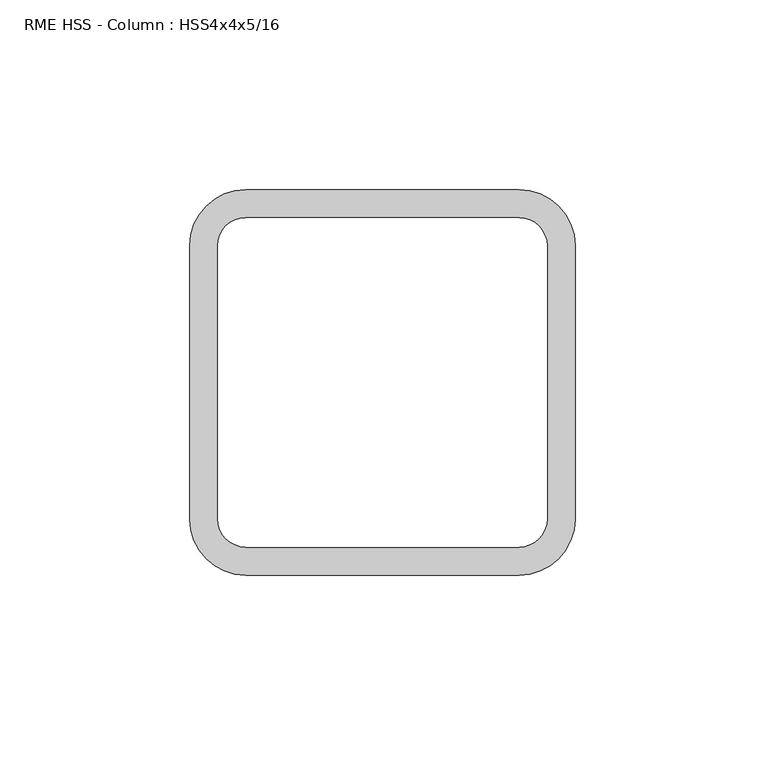
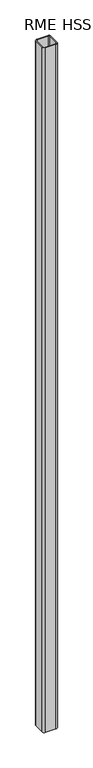
"""IFC4 building model written with IfcOpenShell, lengths in millimetres: column geometry, RME HSS - Column : HSS4x4x5/16."""

import ifcopenshell
import ifcopenshell.guid

model = None  # the IFC model being written
_history = None  # IfcOwnerHistory: only IFC2X3 demands one
_inside = {}  # id of a spatial element -> (the spatial element, [elements in it])
_under = {}  # id of a project, library or spatial element -> (it, [spatial elements below it])
_declared = {}  # id of a project -> (the project, [libraries it declares])
_typed = {}  # id of a type object -> (the type object, [elements of that type])
_made_of = {}  # id of a material, layer set ... -> (it, [elements and type objects made of it])


def new_model(schema):
    """Start an empty IFC model of exactly this schema.

    Asked for "IFC4X3", IfcOpenShell would pick the latest addendum, in which some entities
    have other attributes; the version numbers below select the first issue.
    IFC2X3 requires an IfcOwnerHistory on every rooted entity: one is made here for all.
    """
    global model, _history
    if schema == "IFC4X3":
        model = ifcopenshell.file(schema_version=(4, 3, 0, 0))
    else:
        model = ifcopenshell.file(schema=schema)
    _inside.clear()
    _under.clear()
    _declared.clear()
    _typed.clear()
    _made_of.clear()
    _history = None
    if model.schema == "IFC2X3":
        org = make("IfcOrganization", Name="unknown")
        user = make(
            "IfcPersonAndOrganization",
            ThePerson=make("IfcPerson", FamilyName="unknown"),
            TheOrganization=org,
        )
        app = make(
            "IfcApplication",
            ApplicationDeveloper=org,
            Version="unknown",
            ApplicationFullName="unknown",
            ApplicationIdentifier="unknown",
        )
        _history = make(
            "IfcOwnerHistory",
            OwningUser=user,
            OwningApplication=app,
            ChangeAction="ADDED",
            CreationDate=0,
        )
    return model


def make(cls, **values):
    """One entity of the class cls with the attributes given. An attribute that is None is left unset."""
    return model.create_entity(
        cls, **{name: value for name, value in values.items() if value is not None}
    )


def rooted(cls, **values):
    """An entity with a GlobalId (a new one), such as an element, a storey or a relation."""
    return make(cls, GlobalId=ifcopenshell.guid.new(), OwnerHistory=_history, **values)


def si_unit(unit_type, name, prefix=None):
    """IfcSIUnit, for example si_unit("LENGTHUNIT", "METRE", prefix="MILLI")."""
    return make("IfcSIUnit", UnitType=unit_type, Prefix=prefix, Name=name)


def assignment(units):
    """IfcUnitAssignment: the units of a project."""
    return None if units is None else make("IfcUnitAssignment", Units=units)


def point(xyz):
    """IfcCartesianPoint."""
    return None if xyz is None else make("IfcCartesianPoint", Coordinates=xyz)


def direction(xyz):
    """IfcDirection."""
    return None if xyz is None else make("IfcDirection", DirectionRatios=xyz)


def frame(location, z_axis=None, x_axis=None):
    """IfcAxis2Placement3D, a coordinate frame: its origin and axes. An axis left out is left unset."""
    return make(
        "IfcAxis2Placement3D",
        Location=point(location),
        Axis=direction(z_axis),
        RefDirection=direction(x_axis),
    )


def frame_2d(location, x_axis=None):
    """IfcAxis2Placement2D, a coordinate frame in the plane: its origin and x axis."""
    return make(
        "IfcAxis2Placement2D", Location=point(location), RefDirection=direction(x_axis)
    )


def origin():
    """The frame at (0, 0, 0) with its axes left unset."""
    return frame((0.0, 0.0, 0.0))


def place(relative_to, where):
    """IfcLocalPlacement: puts the frame where relative to a parent placement (None: the world)."""
    return make(
        "IfcLocalPlacement", PlacementRelTo=relative_to, RelativePlacement=where
    )


def context(
    kind, dimensions, precision=None, world=None, true_north=None, identifier=None
):
    """IfcGeometricRepresentationContext, for example the 3D "Model" context."""
    return make(
        "IfcGeometricRepresentationContext",
        ContextIdentifier=identifier,
        ContextType=kind,
        CoordinateSpaceDimension=dimensions,
        Precision=precision,
        WorldCoordinateSystem=world,
        TrueNorth=true_north,
    )


def project(units=None, contexts=None):
    """IfcProject with its units and contexts."""
    return rooted(
        "IfcProject",
        Name="project",
        RepresentationContexts=contexts,
        UnitsInContext=assignment(units),
    )


def spatial(cls, under=None, at=None, **own):
    """A site, building, storey or space (cls), placed at a placement, below another one or the project."""
    s = rooted(cls, ObjectPlacement=at, **own)
    if under is not None:
        _under.setdefault(under.id(), (under, []))[1].append(s)
    return s


def polyline(points):
    """IfcPolyline through the points."""
    return make("IfcPolyline", Points=[point(p) for p in points])


def circle_curve(where, radius):
    """IfcCircle in the frame where."""
    return make("IfcCircle", Position=where, Radius=radius)


def trimmed(basis, trim1, trim2, sense, master):
    """IfcTrimmedCurve: the piece of a basis curve between two trims."""
    return make(
        "IfcTrimmedCurve",
        BasisCurve=basis,
        Trim1=trim1,
        Trim2=trim2,
        SenseAgreement=sense,
        MasterRepresentation=master,
    )


def segment(curve, same_sense, transition):
    """IfcCompositeCurveSegment."""
    return make(
        "IfcCompositeCurveSegment",
        Transition=transition,
        SameSense=same_sense,
        ParentCurve=curve,
    )


def composite_curve(segments, self_intersect=None):
    """IfcCompositeCurve: segments joined end to end."""
    return make("IfcCompositeCurve", Segments=segments, SelfIntersect=self_intersect)


def outline(outer, holes=None, kind="AREA"):
    """IfcArbitraryClosedProfileDef: a profile drawn as a closed curve; with holes, ...WithVoids."""
    if holes is None:
        return make("IfcArbitraryClosedProfileDef", ProfileType=kind, OuterCurve=outer)
    return make(
        "IfcArbitraryProfileDefWithVoids",
        ProfileType=kind,
        OuterCurve=outer,
        InnerCurves=holes,
    )


def extrude(swept, where, along, depth):
    """IfcExtrudedAreaSolid: the profile swept, set in the frame where, extruded along a direction by depth."""
    return make(
        "IfcExtrudedAreaSolid",
        SweptArea=swept,
        Position=where,
        ExtrudedDirection=direction(along),
        Depth=depth,
    )


def shape(context_of_items, identifier, shape_type, items):
    """IfcShapeRepresentation: the items that make up one representation, for example the "Body"."""
    return make(
        "IfcShapeRepresentation",
        ContextOfItems=context_of_items,
        RepresentationIdentifier=identifier,
        RepresentationType=shape_type,
        Items=items,
    )


def source(mapping_origin, context_of_items, identifier, shape_type, items):
    """IfcRepresentationMap: a shape defined once, which mapped items show again and again."""
    return make(
        "IfcRepresentationMap",
        MappingOrigin=mapping_origin,
        MappedRepresentation=shape(context_of_items, identifier, shape_type, items),
    )


def transform(
    local_origin,
    x_axis=None,
    y_axis=None,
    z_axis=None,
    scale=None,
    scale2=None,
    scale3=None,
    uniform=True,
):
    """IfcCartesianTransformationOperator3D, or its non-uniform kind. x_axis, y_axis, z_axis: its Axis1, 2, 3."""
    if uniform:
        return make(
            "IfcCartesianTransformationOperator3D",
            Axis1=direction(x_axis),
            Axis2=direction(y_axis),
            LocalOrigin=point(local_origin),
            Scale=scale,
            Axis3=direction(z_axis),
        )
    return make(
        "IfcCartesianTransformationOperator3DnonUniform",
        Axis1=direction(x_axis),
        Axis2=direction(y_axis),
        LocalOrigin=point(local_origin),
        Scale=scale,
        Axis3=direction(z_axis),
        Scale2=scale2,
        Scale3=scale3,
    )


def mapped(mapping_source, mapping_target):
    """IfcMappedItem: shows the shape of a source again, moved by a transform."""
    return make(
        "IfcMappedItem", MappingSource=mapping_source, MappingTarget=mapping_target
    )


def made_of(thing, what):
    """Note that an element or type object is made of a material, layer set ...; save() writes the relation."""
    if what is not None:
        _made_of.setdefault(what.id(), (what, []))[1].append(thing)
    return thing


def element(
    cls,
    number,
    at=None,
    inside=None,
    cuts=None,
    type_object=None,
    material=None,
    context=None,
    identifier="Body",
    shape_type=None,
    held_by="IfcProductDefinitionShape",
    body=None,
    shapes=None,
    **own,
):
    """One element of the class cls, such as IfcWall. Its Tag is "e" and its number.

    at: its placement. inside: the storey or other place that contains it. cuts: it is an
    opening in that element (IfcRelVoidsElement). A single representation is given by context,
    identifier, shape_type and body (its items); several are given by shapes. held_by: the class
    of the entity that holds the representations. save() writes the other relations.
    """
    e = rooted(cls, Tag="e%d" % number, ObjectPlacement=at, **own)
    if body is not None:
        shapes = [shape(context, identifier, shape_type, body)]
    if shapes is not None:
        e.Representation = make(held_by, Representations=shapes)
    if inside is not None:
        _inside.setdefault(inside.id(), (inside, []))[1].append(e)
    if cuts is not None:
        rooted(
            "IfcRelVoidsElement", RelatingBuildingElement=cuts, RelatedOpeningElement=e
        )
    if type_object is not None:
        _typed.setdefault(type_object.id(), (type_object, []))[1].append(e)
    return made_of(e, material)


def aggregate(whole, parts):
    """IfcRelAggregates: a whole, such as a stair, and the parts it consists of."""
    return rooted("IfcRelAggregates", RelatingObject=whole, RelatedObjects=parts)


def save(model, path):
    """Write the relations noted so far, then the file.

    IfcRelAggregates (storeys below a building ...), IfcRelContainedInSpatialStructure (elements
    in a storey), IfcRelDefinesByType, IfcRelAssociatesMaterial and IfcRelDeclares: one each for
    every whole, place, type object, material and project.
    """
    for whole, parts in _under.values():
        aggregate(whole, parts)
    for where, things in _inside.values():
        rooted(
            "IfcRelContainedInSpatialStructure",
            RelatedElements=things,
            RelatingStructure=where,
        )
    for kind, things in _typed.values():
        rooted("IfcRelDefinesByType", RelatedObjects=things, RelatingType=kind)
    for what, things in _made_of.values():
        rooted("IfcRelAssociatesMaterial", RelatedObjects=things, RelatingMaterial=what)
    for by, libraries in _declared.values():
        rooted("IfcRelDeclares", RelatingContext=by, RelatedDefinitions=libraries)
    model.write(path)


def rme_hss_column_hss4x4x5_16_3b7b5b5a(model_context):
    return source(origin(), model_context, "Body", "SweptSolid", [
        extrude(outline(composite_curve([segment(trimmed(circle_curve(frame_2d((36.0172, 36.0172)), 14.7828), [point((36.0172, 50.8))], [point((50.8, 36.0172))], False, "CARTESIAN"), True, "CONTINUOUS"), segment(polyline([(50.8, 36.0172), (50.8, -36.0172)]), True, "CONTINUOUS"), segment(trimmed(circle_curve(frame_2d((36.0172, -36.0172)), 14.7828), [point((50.8, -36.0172))], [point((36.0172, -50.8))], False, "CARTESIAN"), True, "CONTINUOUS"), segment(polyline([(36.0172, -50.8), (-36.0172, -50.8)]), True, "CONTINUOUS"), segment(trimmed(circle_curve(frame_2d((-36.0172, -36.0172)), 14.7828), [point((-36.0172, -50.8))], [point((-50.8, -36.0172))], False, "CARTESIAN"), True, "CONTINUOUS"), segment(polyline([(-50.8, -36.0172), (-50.8, 36.0172)]), True, "CONTINUOUS"), segment(trimmed(circle_curve(frame_2d((-36.0172, 36.0172)), 14.7828), [point((-50.8, 36.0172))], [point((-36.0172, 50.8))], False, "CARTESIAN"), True, "CONTINUOUS"), segment(polyline([(-36.0172, 50.8), (36.0172, 50.8)]), True, "CONTINUOUS")], self_intersect=False), holes=[composite_curve([segment(polyline([(36.0172, 43.4086), (-36.0172, 43.4086)]), True, "CONTINUOUS"), segment(trimmed(circle_curve(frame_2d((-36.0172, 36.0172)), 7.3914), [point((-36.0172, 43.4086))], [point((-43.4086, 36.0172))], True, "CARTESIAN"), True, "CONTINUOUS"), segment(polyline([(-43.4086, 36.0172), (-43.4086, -36.0172)]), True, "CONTINUOUS"), segment(trimmed(circle_curve(frame_2d((-36.0172, -36.0172)), 7.3914), [point((-43.4086, -36.0172))], [point((-36.0172, -43.4086))], True, "CARTESIAN"), True, "CONTINUOUS"), segment(polyline([(-36.0172, -43.4086), (36.0172, -43.4086)]), True, "CONTINUOUS"), segment(trimmed(circle_curve(frame_2d((36.0172, -36.0172)), 7.3914), [point((36.0172, -43.4086))], [point((43.4086, -36.0172))], True, "CARTESIAN"), True, "CONTINUOUS"), segment(polyline([(43.4086, -36.0172), (43.4086, 36.0172)]), True, "CONTINUOUS"), segment(trimmed(circle_curve(frame_2d((36.0172, 36.0172)), 7.3914), [point((43.4086, 36.0172))], [point((36.0172, 43.4086))], True, "CARTESIAN"), True, "CONTINUOUS")], self_intersect=False)]), frame((0.0, 0.0, -304.8), z_axis=(0.0, 0.0, 1.0), x_axis=(1.0, 0.0, 0.0)), (0.0, 0.0, 1.0), 4902.2),
    ])


if __name__ == "__main__":
    model = new_model("IFC4")
    model_context = context("Model", 3, world=origin())
    ifc_project = project(units=[si_unit("LENGTHUNIT", "METRE", prefix="MILLI")], contexts=[model_context])
    site = spatial("IfcSite", under=ifc_project)
    building = spatial("IfcBuilding", under=site)
    placement = place(None, origin())
    rme_hss_column_hss4x4x5_16_shape = rme_hss_column_hss4x4x5_16_3b7b5b5a(model_context)
    element("IfcColumn", 1, ObjectType="RME HSS - Column : HSS4x4x5/16", at=placement, inside=building, context=model_context, shape_type="MappedRepresentation", body=[
        mapped(rme_hss_column_hss4x4x5_16_shape, transform((0.0, 0.0, 0.0), x_axis=(1.0, 0.0, 0.0), y_axis=(0.0, 1.0, 0.0), z_axis=(0.0, 0.0, 1.0))),
    ])
    save(model, "model.ifc")

# Revit data of these elements
# Type "RME HSS - Column : HSS4x4x5/16"
#   Nominal Size = ""
#   Base Plate Type [instance default] = ""
#   Assembly Code = "B10"
#   Shape = "Square"
#   W = 14.8
#   Ht = 0' - 4"
#   b = 0' - 4"
#   kr = 0' - 0.582"
#   t = 0' - 0.291"
#   A = 0.0284722 SF
#   Structural Material [instance default] = Metal - Steel - ASTM A500 - Grade B - Rectangular and Square
# Element 1 (IfcColumn, "RME HSS - Column : HSS4x4x5/16")
#   Structural Material = Metal - Steel - ASTM A992
#   Materials on its faces: "Metal - Steel - ASTM A992"
# Materials
#   "Metal - Steel - ASTM A500 - Grade B - Rectangular and Square": class "Metal", colour RGB 255 128 0, transparency 0
#   "Metal - Steel - ASTM A992": class "Metal", colour RGB 255 128 0, transparency 0
